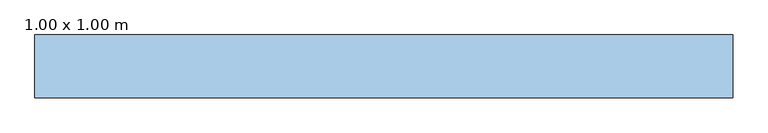
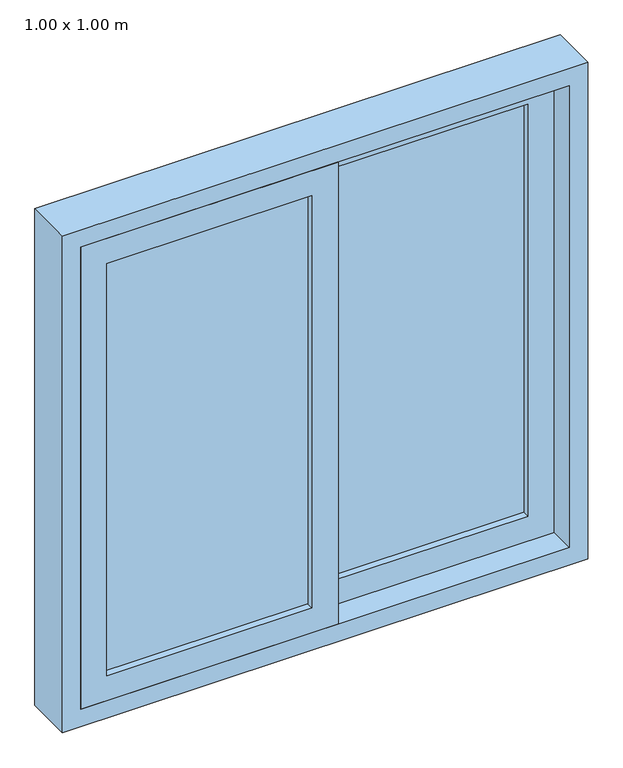
"""IFC4 building model written with IfcOpenShell, lengths in millimetres: window geometry, Janela de correr vidro - 2 Folhas : 1.00 x 1.00 m."""

from ifc_helpers import new_model, si_unit, frame, origin, place, context, project, spatial, polyline, outline, extrude, source, transform, mapped, element, save


def window_1_00_x_1_00_m_519e731f(model_context):
    return source(origin(), model_context, "Body", "SweptSolid", [
        extrude(outline(polyline([(935.0, -25.0), (935.0, 465.0), (1865.0, 465.0), (1865.0, -25.0), (935.0, -25.0)]), holes=[polyline([(1815.0, 25.0), (1815.0, 415.0), (985.0, 415.0), (985.0, 25.0), (1815.0, 25.0)])]), frame((0.0, -35.0, 0.0), z_axis=(0.0, 1.0, 0.0), x_axis=(0.0, 0.0, 1.0)), (0.0, 0.0, 1.0), 40.0),
        extrude(outline(polyline([(1865.0, 25.0), (1865.0, -465.0), (935.0, -465.0), (935.0, 25.0), (1865.0, 25.0)]), holes=[polyline([(985.0, -25.0), (985.0, -415.0), (1815.0, -415.0), (1815.0, -25.0), (985.0, -25.0)])]), frame((0.0, -85.0, 0.0), z_axis=(0.0, 1.0, 0.0), x_axis=(0.0, 0.0, 1.0)), (0.0, 0.0, 1.0), 40.0),
        extrude(outline(polyline([(1900.0, 500.0), (1900.0, -500.0), (900.0, -500.0), (900.0, 500.0), (1900.0, 500.0)]), holes=[polyline([(935.0, 465.0), (935.0, -465.0), (1865.0, -465.0), (1865.0, 465.0), (935.0, 465.0)])]), frame((0.0, -85.0, 0.0), z_axis=(0.0, 1.0, 0.0), x_axis=(0.0, 0.0, 1.0)), (0.0, 0.0, 1.0), 90.0),
        extrude(outline(polyline([(25.0, -8.0), (415.0, -8.0), (415.0, -22.0), (25.0, -22.0), (25.0, -8.0)])), frame((0.0, 0.0, 985.0), z_axis=(0.0, 0.0, 1.0), x_axis=(1.0, 0.0, 0.0)), (0.0, 0.0, 1.0), 830.0),
        extrude(outline(polyline([(-415.0, -58.0), (-25.0, -58.0), (-25.0, -72.0), (-415.0, -72.0), (-415.0, -58.0)])), frame((0.0, 0.0, 985.0), z_axis=(0.0, 0.0, 1.0), x_axis=(1.0, 0.0, 0.0)), (0.0, 0.0, 1.0), 830.0),
    ])


if __name__ == "__main__":
    model = new_model("IFC4")
    model_context = context("Model", 3, world=origin())
    ifc_project = project(units=[si_unit("LENGTHUNIT", "METRE", prefix="MILLI")], contexts=[model_context])
    site = spatial("IfcSite", under=ifc_project)
    building = spatial("IfcBuilding", under=site)
    placement = place(None, origin())
    window_1_00_x_1_00_m_shape = window_1_00_x_1_00_m_519e731f(model_context)
    element("IfcWindow", 1, ObjectType="Janela de correr vidro - 2 Folhas : 1.00 x 1.00 m", at=placement, inside=building, context=model_context, shape_type="MappedRepresentation", body=[
        mapped(window_1_00_x_1_00_m_shape, transform((0.0, 0.0, 0.0), x_axis=(1.0, 0.0, 0.0), y_axis=(0.0, 1.0, 0.0), z_axis=(0.0, 0.0, 1.0))),
    ])
    save(model, "model.ifc")

# Revit data of these elements
# Project information
#   Data de emissão do projeto = "Data de emissão"
#   Status do projeto = "Status do projeto"
#   Nome do cliente = "Proprietário"
#   Endereço do projeto = "RUA A - BLOCO A"
#   Nome do projeto = "CURSO REVIT PLANTA HUMANIZADA"
#   Número do projeto = "Número do projeto"
# Type "Janela de correr vidro - 2 Folhas : 1.00 x 1.00 m"
#   Type Mark = "J26"
#   Construction Type Id = "GSP4R"
#   Analytic Construction = "Vidraça única Pilkington 1/8 pol"
#   Visual Light Transmittance = 0.9
#   Thermal Resistance (R) = 0.271106 (m²·K)/W
#   Solar Heat Gain Coefficient = 0.78
#   Rough Width = 1.000 m
#   Rough Height = 1.000 m
#   Largura da moldura do painel = 0.050 m
#   Espessura da moldura do painel = 0.040 m
#   Height = 1.000 m
#   Heat Transfer Coefficient (U) = 3.6886 W/(m²·K)
#   Largura da estrutura = 0.035 m
#   Espessura da moldura = 0.090 m
#   Altura-padrão do peitoril = 0.900 m
#   Width = 1.000 m
#   Pingadeira = yes
#   Material da Pingadeira = Granito amarelo
#   Vidro = Vidro
#   Material da estrutura = Metal - Alumínio
#   Wall Closure = (empty or 0)
# Element 1 (IfcWindow, "Janela de correr vidro - 2 Folhas : 1.00 x 1.00 m")
#   Materials on its faces: "Metal - Alumínio", "Vidro"
# Materials
#   "Granito amarelo": class "Genérico", colour RGB 80 80 80, transparency 0, Cost = 0
#   "Vidro": class "Vidro", colour RGB 0 128 192, transparency 0.9
#   "Metal - Alumínio": class "Metal", colour RGB 247 247 247, transparency 0
